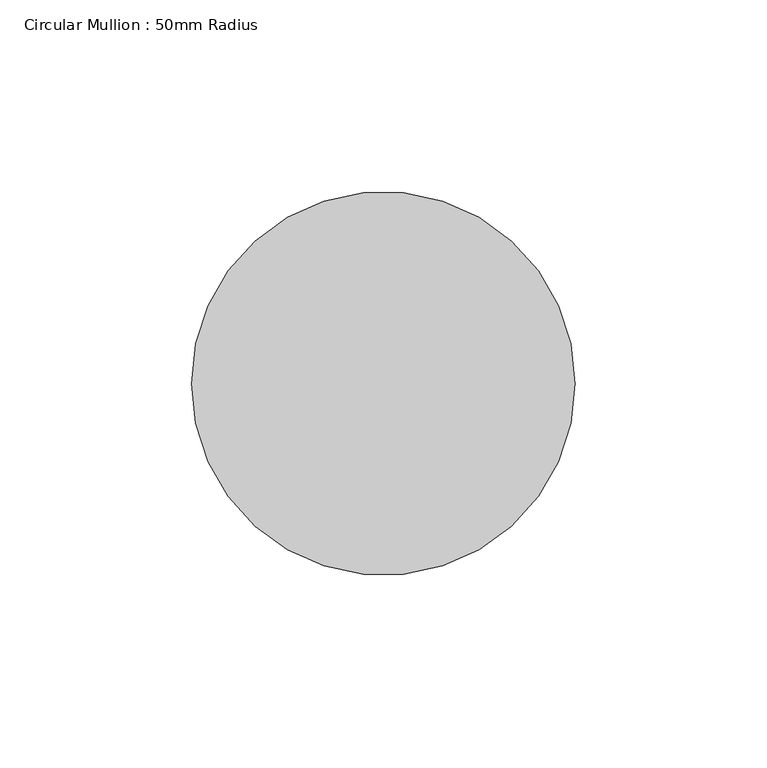
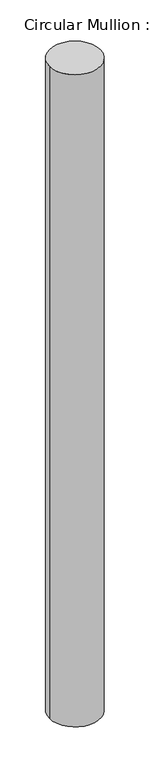
"""IFC4 building model written with IfcOpenShell, lengths in millimetres: member geometry, Circular Mullion : 50mm Radius."""

from ifc_helpers import new_model, si_unit, point, frame, origin, origin_2d, place, context, project, spatial, circle_curve, trimmed, segment, composite_curve, outline, extrude, source, transform, mapped, element, save


def circular_mullion_50mm_radius_f77dbb90(model_context):
    return source(origin(), model_context, "Body", "SweptSolid", [
        extrude(outline(composite_curve([segment(trimmed(circle_curve(origin_2d(), 50.0), [point((50.0, 0.0))], [point((-50.0, 0.0))], False, "CARTESIAN"), True, "CONTINUOUS"), segment(trimmed(circle_curve(origin_2d(), 50.0), [point((-50.0, 0.0))], [point((50.0, 0.0))], False, "CARTESIAN"), True, "CONTINUOUS")], self_intersect=False)), frame((0.0, 0.0, -1351.9895086), z_axis=(0.0, 0.0, 1.0), x_axis=(1.0, 0.0, 0.0)), (0.0, 0.0, 1.0), 1351.9895086),
    ])


if __name__ == "__main__":
    model = new_model("IFC4")
    model_context = context("Model", 3, world=origin())
    ifc_project = project(units=[si_unit("LENGTHUNIT", "METRE", prefix="MILLI")], contexts=[model_context])
    site = spatial("IfcSite", under=ifc_project)
    building = spatial("IfcBuilding", under=site)
    placement = place(None, origin())
    circular_mullion_50mm_radius_shape = circular_mullion_50mm_radius_f77dbb90(model_context)
    element("IfcMember", 1, ObjectType="Circular Mullion : 50mm Radius", at=placement, inside=building, context=model_context, shape_type="MappedRepresentation", body=[
        mapped(circular_mullion_50mm_radius_shape, transform((0.0, 0.0, 0.0), x_axis=(1.0, 0.0, 0.0), y_axis=(0.0, 1.0, 0.0), z_axis=(0.0, 0.0, 1.0))),
    ])
    save(model, "model.ifc")

# Revit data of these elements
# Type "Circular Mullion : 50mm Radius"
#   built-in parameter 1007350 = 0.164042 (stored number, unit not read)
# Element 1 (IfcMember, "Circular Mullion : 50mm Radius")
#   Materials on its faces: "Aluminium"
# Materials
#   "Aluminium": class "Metal", colour RGB 247 247 247, transparency 0, Description = "Aluminium 6061", Cost = 0
